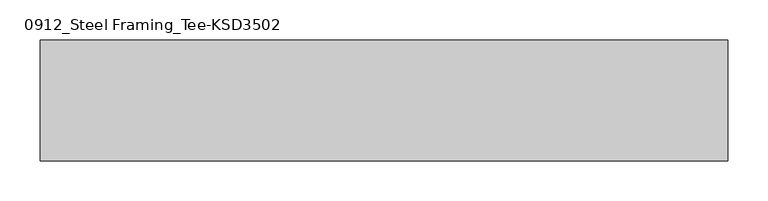
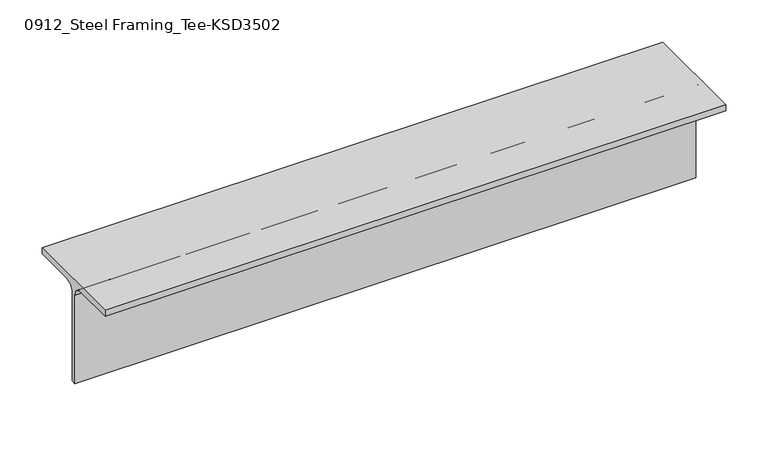
"""IFC4 building model written with IfcOpenShell, lengths in millimetres: member geometry, 0912_Steel Framing_Tee-KSD3502 : H_SB_ASB_CT-150x150x6.5x9."""

from ifc_helpers import new_model, si_unit, point, frame, frame_2d, origin, place, context, project, spatial, polyline, circle_curve, trimmed, segment, composite_curve, outline, extrude, source, transform, mapped, element, save


def member_0912_steel_framing_tee_ksd3502_558173c0(model_context):
    return source(origin(), model_context, "Body", "SweptSolid", [
        extrude(outline(composite_curve([segment(polyline([(-75.0, 75.0), (75.0, 75.0), (75.0, 66.0), (16.25, 66.0)]), True, "CONTINUOUS"), segment(trimmed(circle_curve(frame_2d((16.25, 53.0)), 13.0), [point((16.25, 66.0))], [point((3.25, 53.0))], True, "CARTESIAN"), True, "CONTINUOUS"), segment(polyline([(3.25, 53.0), (3.25, -75.0), (-3.25, -75.0), (-3.25, 53.0)]), True, "CONTINUOUS"), segment(trimmed(circle_curve(frame_2d((-16.25, 53.0)), 13.0), [point((-3.25, 53.0))], [point((-16.25, 66.0))], True, "CARTESIAN"), True, "CONTINUOUS"), segment(polyline([(-16.25, 66.0), (-75.0, 66.0), (-75.0, 75.0)]), True, "CONTINUOUS")], self_intersect=False)), frame((-353.0, 0.0, 0.0), z_axis=(1.0, 0.0, 0.0), x_axis=(0.0, 1.0, 0.0)), (0.0, 0.0, 1.0), 853.0),
    ])


if __name__ == "__main__":
    model = new_model("IFC4")
    model_context = context("Model", 3, world=origin())
    ifc_project = project(units=[si_unit("LENGTHUNIT", "METRE", prefix="MILLI")], contexts=[model_context])
    site = spatial("IfcSite", under=ifc_project)
    building = spatial("IfcBuilding", under=site)
    placement = place(None, origin())
    member_0912_steel_framing_tee_ksd3502_shape = member_0912_steel_framing_tee_ksd3502_558173c0(model_context)
    element("IfcMember", 1, ObjectType="0912_Steel Framing_Tee-KSD3502 : H_SB_ASB_CT-150x150x6.5x9", at=placement, inside=building, context=model_context, shape_type="MappedRepresentation", body=[
        mapped(member_0912_steel_framing_tee_ksd3502_shape, transform((0.0, 0.0, 0.0), x_axis=(1.0, 0.0, 0.0), y_axis=(0.0, 1.0, 0.0), z_axis=(0.0, 0.0, 1.0))),
    ])
    save(model, "model.ifc")

# Revit data of these elements
# Type "0912_Steel Framing_Tee-KSD3502 : H_SB_ASB_CT-150x150x6.5x9"
#   H_WM Code_1 = "S01AA003-00001 | Main Steel Structure Fabrication Work | Shelter/Building | Light Steel - Standard (30KG/M>Weight) | Material: (   )"
#   H_WM Code_2 = "S03AA029-00001 | Main Steel Structure Erection Work | Shelter/Building | Light Steel (30KG/M>Weight) | Material: (   )"
#   H_WM Code_3 = "S01AA010-00001 | Main Steel Structure Fabrication Work | Shelter/Building | Steel Painting/Coating | for Non-Fireproofed Steel Surface, Surface Preparation, Primer, Second & Final Coat | Material: (   )"
#   H_Q'ty Cal Type Tag = "SB-Q2"
#   Width = 15.0 cm
#   Web Thickness = 0.65 cm
#   Web Fillet = 1.3 cm
#   Section Area = 23.39 cm²
#   Perimeter = 0.60 m²/m
#   Nominal Weight = 18.40 kgf/m
#   Height = 15.0 cm
#   Flange Thickness = 0.9 cm
#   Centroid Vertical = 7.5 cm
#   Centroid Horizontal = 7.5 cm
#   Length [instance default] = 1.5000 m
#   Structural Material [instance default] = Steel, 45-345
#   Warping Constant = (empty or 0)
#   Torsional Moment of Inertia = 0
#   Section Name Key = ""
#   Plastic Modulus weak axis = 0
#   Plastic Modulus strong axis = 0
#   Moment of Inertia weak axis = 0
#   Moment of Inertia strong axis = 0
#   Elastic Modulus weak axis = 0
#   Elastic Modulus strong axis = 0
#   Bolt Spacing = 0
#   Assembly Code = ""
# Element 1 (IfcMember, "0912_Steel Framing_Tee-KSD3502 : H_SB_ASB_CT-150x150x6.5x9")
#   Structural Material = none
# Materials
#   "Steel, 45-345": class "Metal", colour RGB 189 187 185, transparency 0, Description = "Steel 345 MPa", Cost = 0
